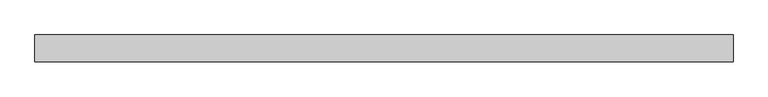
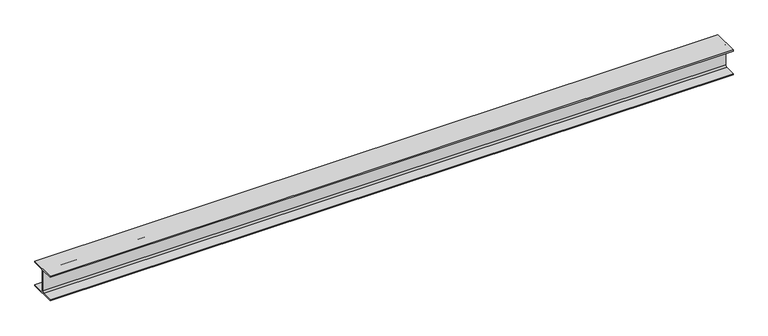
"""IFC4 building model written with IfcOpenShell, lengths in millimetres: beam geometry, 0912_Steel Framing_H-KSD3502 : H_SB_ASB_H-300x300x10x15."""

from ifc_helpers import new_model, si_unit, point, frame, frame_2d, origin, place, context, project, spatial, polyline, circle_curve, trimmed, segment, composite_curve, outline, extrude, source, transform, mapped, element, save


def beam_8c8e336d(model_context):
    return source(origin(), model_context, "Body", "SweptSolid", [
        extrude(outline(composite_curve([segment(polyline([(150.0, -135.0), (150.0, -150.0), (-150.0, -150.0), (-150.0, -135.0), (-23.0, -135.0)]), True, "CONTINUOUS"), segment(trimmed(circle_curve(frame_2d((-23.0, -117.0)), 18.0), [point((-23.0, -135.0))], [point((-5.0, -117.0))], True, "CARTESIAN"), True, "CONTINUOUS"), segment(polyline([(-5.0, -117.0), (-5.0, 117.0)]), True, "CONTINUOUS"), segment(trimmed(circle_curve(frame_2d((-23.0, 117.0)), 18.0), [point((-5.0, 117.0))], [point((-23.0, 135.0))], True, "CARTESIAN"), True, "CONTINUOUS"), segment(polyline([(-23.0, 135.0), (-150.0, 135.0), (-150.0, 150.0), (150.0, 150.0), (150.0, 135.0), (23.0, 135.0)]), True, "CONTINUOUS"), segment(trimmed(circle_curve(frame_2d((23.0, 117.0)), 18.0), [point((23.0, 135.0))], [point((5.0, 117.0))], True, "CARTESIAN"), True, "CONTINUOUS"), segment(polyline([(5.0, 117.0), (5.0, -117.0)]), True, "CONTINUOUS"), segment(trimmed(circle_curve(frame_2d((23.0, -117.0)), 18.0), [point((5.0, -117.0))], [point((23.0, -135.0))], True, "CARTESIAN"), True, "CONTINUOUS"), segment(polyline([(23.0, -135.0), (150.0, -135.0)]), True, "CONTINUOUS")], self_intersect=False)), frame((-4027.4502484, 0.0, 0.0), z_axis=(1.0, 0.0, 0.0), x_axis=(0.0, 1.0, 0.0)), (0.0, 0.0, 1.0), 7805.3816456),
    ])


if __name__ == "__main__":
    model = new_model("IFC4")
    model_context = context("Model", 3, world=origin())
    ifc_project = project(units=[si_unit("LENGTHUNIT", "METRE", prefix="MILLI")], contexts=[model_context])
    site = spatial("IfcSite", under=ifc_project)
    building = spatial("IfcBuilding", under=site)
    placement = place(None, origin())
    beam_shape = beam_8c8e336d(model_context)
    element("IfcBeam", 1, ObjectType="0912_Steel Framing_H-KSD3502 : H_SB_ASB_H-300x300x10x15", at=placement, inside=building, context=model_context, shape_type="MappedRepresentation", body=[
        mapped(beam_shape, transform((0.0, 0.0, 0.0), x_axis=(1.0, 0.0, 0.0), y_axis=(0.0, 1.0, 0.0), z_axis=(0.0, 0.0, 1.0))),
    ])
    save(model, "model.ifc")

# Revit data of these elements
# Type "0912_Steel Framing_H-KSD3502 : H_SB_ASB_H-300x300x10x15"
#   H_WM Code_1 = "S01AA001-00001 | Main Steel Structure Fabrication Work | Shelter/Building | Heavy Steel - Standard (Weight≥90KG/M) | Material: (   )"
#   H_WM Code_2 = "S03AA027-00001 | Main Steel Structure Erection Work | Shelter/Building | Heavy Steel (Weight≥90KG/M) | Material: (   )"
#   H_WM Code_3 = "S01AA010-00001 | Main Steel Structure Fabrication Work | Shelter/Building | Steel Painting/Coating | for Non-Fireproofed Steel Surface, Surface Preparation, Primer, Second & Final Coat | Material: (   )"
#   H_Q'ty Cal Type Tag = "SB-Q2"
#   Width = 30.0 cm
#   Web Thickness = 1.0 cm
#   Web Fillet = 1.8 cm
#   Warping Constant = 1370000.0 cm⁶
#   W = 0
#   Torsional Moment of Inertia = 77.00 cm⁴
#   Section Area = 119.8 cm²
#   Plastic Modulus weak axis = 684.0 cm³
#   Plastic Modulus strong axis = 1500.0 cm³
#   Perimeter = 1.75 m²/m
#   Nominal Weight = 94.00 kgf/m
#   Moment of Inertia weak axis = 6750.00 cm⁴
#   Moment of Inertia strong axis = 20400.00 cm⁴
#   Height = 30.0 cm
#   Flange Thickness = 1.5 cm
#   Elastic Modulus weak axis = 450.0 cm³
#   Elastic Modulus strong axis = 1360.0 cm³
#   Centroid Vertical = 15.0 cm
#   Centroid Horizontal = 15.0 cm
#   Ix = 204000000
#   Length [instance default] = 1.5240 m
#   Zx = 1500000
#   b = 0.3000 m
#   h = 0.3000 m
#   r = 0.0180 m
#   s = 0.0100 m
#   t = 0.0150 m
#   A = 0.01198 m²
#   Structural Material [instance default] = Steel, 45-345
#   Assembly Code = ""
# Element 1 (IfcBeam, "0912_Steel Framing_H-KSD3502 : H_SB_ASB_H-300x300x10x15")
#   Structural Material = none
# Materials
#   "Steel, 45-345": class "Metal", colour RGB 189 187 185, transparency 0, Description = "Steel 345 MPa", Cost = 0
